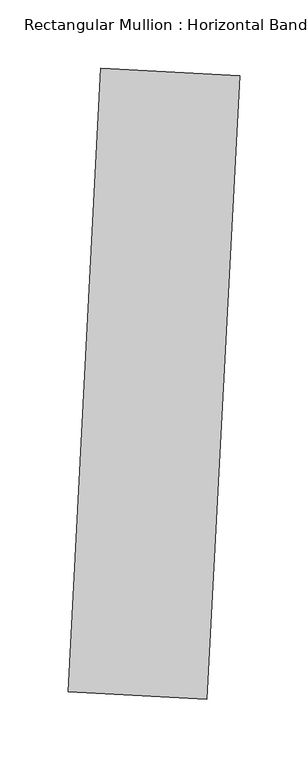
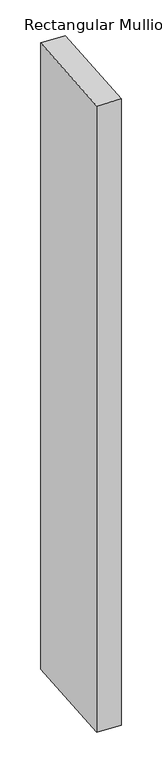
"""IFC4 building model written with IfcOpenShell, lengths in millimetres: member geometry, Rectangular Mullion : Horizontal Band."""

import ifcopenshell
import ifcopenshell.guid

model = None  # the IFC model being written
_history = None  # IfcOwnerHistory: only IFC2X3 demands one
_inside = {}  # id of a spatial element -> (the spatial element, [elements in it])
_under = {}  # id of a project, library or spatial element -> (it, [spatial elements below it])
_declared = {}  # id of a project -> (the project, [libraries it declares])
_typed = {}  # id of a type object -> (the type object, [elements of that type])
_made_of = {}  # id of a material, layer set ... -> (it, [elements and type objects made of it])


def new_model(schema):
    """Start an empty IFC model of exactly this schema.

    Asked for "IFC4X3", IfcOpenShell would pick the latest addendum, in which some entities
    have other attributes; the version numbers below select the first issue.
    IFC2X3 requires an IfcOwnerHistory on every rooted entity: one is made here for all.
    """
    global model, _history
    if schema == "IFC4X3":
        model = ifcopenshell.file(schema_version=(4, 3, 0, 0))
    else:
        model = ifcopenshell.file(schema=schema)
    _inside.clear()
    _under.clear()
    _declared.clear()
    _typed.clear()
    _made_of.clear()
    _history = None
    if model.schema == "IFC2X3":
        org = make("IfcOrganization", Name="unknown")
        user = make(
            "IfcPersonAndOrganization",
            ThePerson=make("IfcPerson", FamilyName="unknown"),
            TheOrganization=org,
        )
        app = make(
            "IfcApplication",
            ApplicationDeveloper=org,
            Version="unknown",
            ApplicationFullName="unknown",
            ApplicationIdentifier="unknown",
        )
        _history = make(
            "IfcOwnerHistory",
            OwningUser=user,
            OwningApplication=app,
            ChangeAction="ADDED",
            CreationDate=0,
        )
    return model


def make(cls, **values):
    """One entity of the class cls with the attributes given. An attribute that is None is left unset."""
    return model.create_entity(
        cls, **{name: value for name, value in values.items() if value is not None}
    )


def rooted(cls, **values):
    """An entity with a GlobalId (a new one), such as an element, a storey or a relation."""
    return make(cls, GlobalId=ifcopenshell.guid.new(), OwnerHistory=_history, **values)


def si_unit(unit_type, name, prefix=None):
    """IfcSIUnit, for example si_unit("LENGTHUNIT", "METRE", prefix="MILLI")."""
    return make("IfcSIUnit", UnitType=unit_type, Prefix=prefix, Name=name)


def assignment(units):
    """IfcUnitAssignment: the units of a project."""
    return None if units is None else make("IfcUnitAssignment", Units=units)


def point(xyz):
    """IfcCartesianPoint."""
    return None if xyz is None else make("IfcCartesianPoint", Coordinates=xyz)


def direction(xyz):
    """IfcDirection."""
    return None if xyz is None else make("IfcDirection", DirectionRatios=xyz)


def frame(location, z_axis=None, x_axis=None):
    """IfcAxis2Placement3D, a coordinate frame: its origin and axes. An axis left out is left unset."""
    return make(
        "IfcAxis2Placement3D",
        Location=point(location),
        Axis=direction(z_axis),
        RefDirection=direction(x_axis),
    )


def origin():
    """The frame at (0, 0, 0) with its axes left unset."""
    return frame((0.0, 0.0, 0.0))


def place(relative_to, where):
    """IfcLocalPlacement: puts the frame where relative to a parent placement (None: the world)."""
    return make(
        "IfcLocalPlacement", PlacementRelTo=relative_to, RelativePlacement=where
    )


def context(
    kind, dimensions, precision=None, world=None, true_north=None, identifier=None
):
    """IfcGeometricRepresentationContext, for example the 3D "Model" context."""
    return make(
        "IfcGeometricRepresentationContext",
        ContextIdentifier=identifier,
        ContextType=kind,
        CoordinateSpaceDimension=dimensions,
        Precision=precision,
        WorldCoordinateSystem=world,
        TrueNorth=true_north,
    )


def project(units=None, contexts=None):
    """IfcProject with its units and contexts."""
    return rooted(
        "IfcProject",
        Name="project",
        RepresentationContexts=contexts,
        UnitsInContext=assignment(units),
    )


def spatial(cls, under=None, at=None, **own):
    """A site, building, storey or space (cls), placed at a placement, below another one or the project."""
    s = rooted(cls, ObjectPlacement=at, **own)
    if under is not None:
        _under.setdefault(under.id(), (under, []))[1].append(s)
    return s


def polyline(points):
    """IfcPolyline through the points."""
    return make("IfcPolyline", Points=[point(p) for p in points])


def outline(outer, holes=None, kind="AREA"):
    """IfcArbitraryClosedProfileDef: a profile drawn as a closed curve; with holes, ...WithVoids."""
    if holes is None:
        return make("IfcArbitraryClosedProfileDef", ProfileType=kind, OuterCurve=outer)
    return make(
        "IfcArbitraryProfileDefWithVoids",
        ProfileType=kind,
        OuterCurve=outer,
        InnerCurves=holes,
    )


def extrude(swept, where, along, depth):
    """IfcExtrudedAreaSolid: the profile swept, set in the frame where, extruded along a direction by depth."""
    return make(
        "IfcExtrudedAreaSolid",
        SweptArea=swept,
        Position=where,
        ExtrudedDirection=direction(along),
        Depth=depth,
    )


def shape(context_of_items, identifier, shape_type, items):
    """IfcShapeRepresentation: the items that make up one representation, for example the "Body"."""
    return make(
        "IfcShapeRepresentation",
        ContextOfItems=context_of_items,
        RepresentationIdentifier=identifier,
        RepresentationType=shape_type,
        Items=items,
    )


def source(mapping_origin, context_of_items, identifier, shape_type, items):
    """IfcRepresentationMap: a shape defined once, which mapped items show again and again."""
    return make(
        "IfcRepresentationMap",
        MappingOrigin=mapping_origin,
        MappedRepresentation=shape(context_of_items, identifier, shape_type, items),
    )


def transform(
    local_origin,
    x_axis=None,
    y_axis=None,
    z_axis=None,
    scale=None,
    scale2=None,
    scale3=None,
    uniform=True,
):
    """IfcCartesianTransformationOperator3D, or its non-uniform kind. x_axis, y_axis, z_axis: its Axis1, 2, 3."""
    if uniform:
        return make(
            "IfcCartesianTransformationOperator3D",
            Axis1=direction(x_axis),
            Axis2=direction(y_axis),
            LocalOrigin=point(local_origin),
            Scale=scale,
            Axis3=direction(z_axis),
        )
    return make(
        "IfcCartesianTransformationOperator3DnonUniform",
        Axis1=direction(x_axis),
        Axis2=direction(y_axis),
        LocalOrigin=point(local_origin),
        Scale=scale,
        Axis3=direction(z_axis),
        Scale2=scale2,
        Scale3=scale3,
    )


def mapped(mapping_source, mapping_target):
    """IfcMappedItem: shows the shape of a source again, moved by a transform."""
    return make(
        "IfcMappedItem", MappingSource=mapping_source, MappingTarget=mapping_target
    )


def made_of(thing, what):
    """Note that an element or type object is made of a material, layer set ...; save() writes the relation."""
    if what is not None:
        _made_of.setdefault(what.id(), (what, []))[1].append(thing)
    return thing


def element(
    cls,
    number,
    at=None,
    inside=None,
    cuts=None,
    type_object=None,
    material=None,
    context=None,
    identifier="Body",
    shape_type=None,
    held_by="IfcProductDefinitionShape",
    body=None,
    shapes=None,
    **own,
):
    """One element of the class cls, such as IfcWall. Its Tag is "e" and its number.

    at: its placement. inside: the storey or other place that contains it. cuts: it is an
    opening in that element (IfcRelVoidsElement). A single representation is given by context,
    identifier, shape_type and body (its items); several are given by shapes. held_by: the class
    of the entity that holds the representations. save() writes the other relations.
    """
    e = rooted(cls, Tag="e%d" % number, ObjectPlacement=at, **own)
    if body is not None:
        shapes = [shape(context, identifier, shape_type, body)]
    if shapes is not None:
        e.Representation = make(held_by, Representations=shapes)
    if inside is not None:
        _inside.setdefault(inside.id(), (inside, []))[1].append(e)
    if cuts is not None:
        rooted(
            "IfcRelVoidsElement", RelatingBuildingElement=cuts, RelatedOpeningElement=e
        )
    if type_object is not None:
        _typed.setdefault(type_object.id(), (type_object, []))[1].append(e)
    return made_of(e, material)


def aggregate(whole, parts):
    """IfcRelAggregates: a whole, such as a stair, and the parts it consists of."""
    return rooted("IfcRelAggregates", RelatingObject=whole, RelatedObjects=parts)


def save(model, path):
    """Write the relations noted so far, then the file.

    IfcRelAggregates (storeys below a building ...), IfcRelContainedInSpatialStructure (elements
    in a storey), IfcRelDefinesByType, IfcRelAssociatesMaterial and IfcRelDeclares: one each for
    every whole, place, type object, material and project.
    """
    for whole, parts in _under.values():
        aggregate(whole, parts)
    for where, things in _inside.values():
        rooted(
            "IfcRelContainedInSpatialStructure",
            RelatedElements=things,
            RelatingStructure=where,
        )
    for kind, things in _typed.values():
        rooted("IfcRelDefinesByType", RelatedObjects=things, RelatingType=kind)
    for what, things in _made_of.values():
        rooted("IfcRelAssociatesMaterial", RelatedObjects=things, RelatingMaterial=what)
    for by, libraries in _declared.values():
        rooted("IfcRelDeclares", RelatingContext=by, RelatedDefinitions=libraries)
    model.write(path)


def rectangular_mullion_horizontal_band_291f11ce(model_context):
    return source(origin(), model_context, "Body", "SweptSolid", [
        extrude(outline(polyline([(62.69438, 301.8280451), (38.7663808, -154.7453782), (-62.69438, -149.4280451), (-38.7663808, 307.1453782), (62.69438, 301.8280451)])), frame((0.0, 0.0, -2820.8179936), z_axis=(0.0, 0.0, 1.0), x_axis=(1.0, 0.0, 0.0)), (0.0, 0.0, 1.0), 2820.8179936),
    ])


if __name__ == "__main__":
    model = new_model("IFC4")
    model_context = context("Model", 3, world=origin())
    ifc_project = project(units=[si_unit("LENGTHUNIT", "METRE", prefix="MILLI")], contexts=[model_context])
    site = spatial("IfcSite", under=ifc_project)
    building = spatial("IfcBuilding", under=site)
    placement = place(None, origin())
    rectangular_mullion_horizontal_band_shape = rectangular_mullion_horizontal_band_291f11ce(model_context)
    element("IfcMember", 1, ObjectType="Rectangular Mullion : Horizontal Band", at=placement, inside=building, context=model_context, shape_type="MappedRepresentation", body=[
        mapped(rectangular_mullion_horizontal_band_shape, transform((0.0, 0.0, 0.0), x_axis=(1.0, 0.0, 0.0), y_axis=(0.0, 1.0, 0.0), z_axis=(0.0, 0.0, 1.0))),
    ])
    save(model, "model.ifc")

# Revit data of these elements
# Type "Rectangular Mullion : Horizontal Band"
#   built-in parameter 1007351 = 0.25 (stored number, unit not read)
#   built-in parameter 1007304 = 1.5 (stored number, unit not read)
#   built-in parameter 1007301 = 0.166667 (stored number, unit not read)
#   built-in parameter 1007300 = 0.166667 (stored number, unit not read)
# Element 1 (IfcMember, "Rectangular Mullion : Horizontal Band")
#   Materials on its faces: "Aluminum"
# Materials
#   "Aluminum": class "Metal", colour RGB 247 247 247, transparency 0, Description = "Aluminum 6061", Cost = 0
